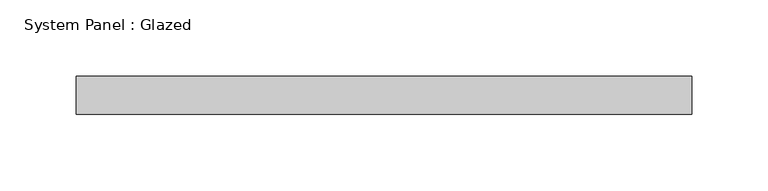
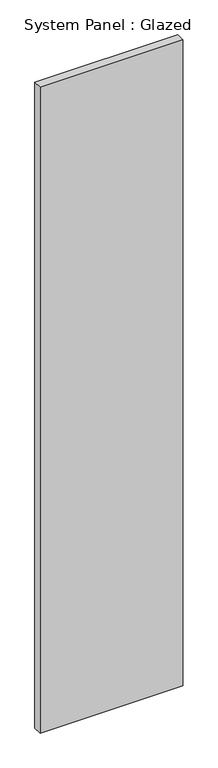
"""IFC4 building model written with IfcOpenShell, lengths in millimetres: plate geometry, System Panel : Glazed."""

from ifc_helpers import new_model, si_unit, origin, origin_with_axes, place, context, project, spatial, polyline, outline, extrude, source, transform, mapped, element, save


def system_panel_glazed_ebe65619(model_context):
    return source(origin(), model_context, "Body", "SweptSolid", [
        extrude(outline(polyline([(202.1619426, -49.5), (-202.1619426, -49.5), (-202.1619426, -24.5), (202.1619426, -24.5), (202.1619426, -49.5)])), origin_with_axes(), (0.0, 0.0, 1.0), 1934.1016494),
    ])


if __name__ == "__main__":
    model = new_model("IFC4")
    model_context = context("Model", 3, world=origin())
    ifc_project = project(units=[si_unit("LENGTHUNIT", "METRE", prefix="MILLI")], contexts=[model_context])
    site = spatial("IfcSite", under=ifc_project)
    building = spatial("IfcBuilding", under=site)
    placement = place(None, origin())
    system_panel_glazed_shape = system_panel_glazed_ebe65619(model_context)
    element("IfcPlate", 1, ObjectType="System Panel : Glazed", at=placement, inside=building, context=model_context, shape_type="MappedRepresentation", body=[
        mapped(system_panel_glazed_shape, transform((0.0, 0.0, 0.0), x_axis=(1.0, 0.0, 0.0), y_axis=(0.0, 1.0, 0.0), z_axis=(0.0, 0.0, 1.0))),
    ])
    save(model, "model.ifc")

# Revit data of these elements
# Type "System Panel : Glazed"
#   Keynote = "H11"
#   Construction Type Id = "GSP4R"
#   Analytic Construction = "1/8 in Pilkington single glazing"
#   Visual Light Transmittance = 0.9
#   Solar Heat Gain Coefficient = 0.86
#   Heat Transfer Coefficient (U) = 6.7069 W/(m²·K)
#   Define Thermal Properties by = 1
# Element 1 (IfcPlate, "System Panel : Glazed")
#   Materials on its faces: "Glass"
# Materials
#   "Glass": class "Glass", colour RGB 0 128 192, transparency 0.9, Description = "Soda Lime Glass", Cost = 0
